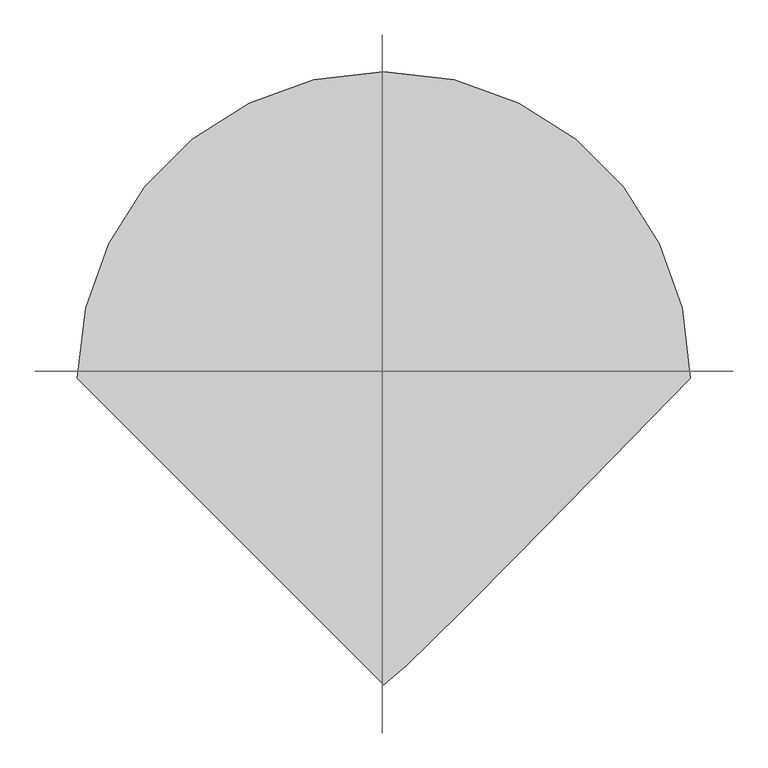
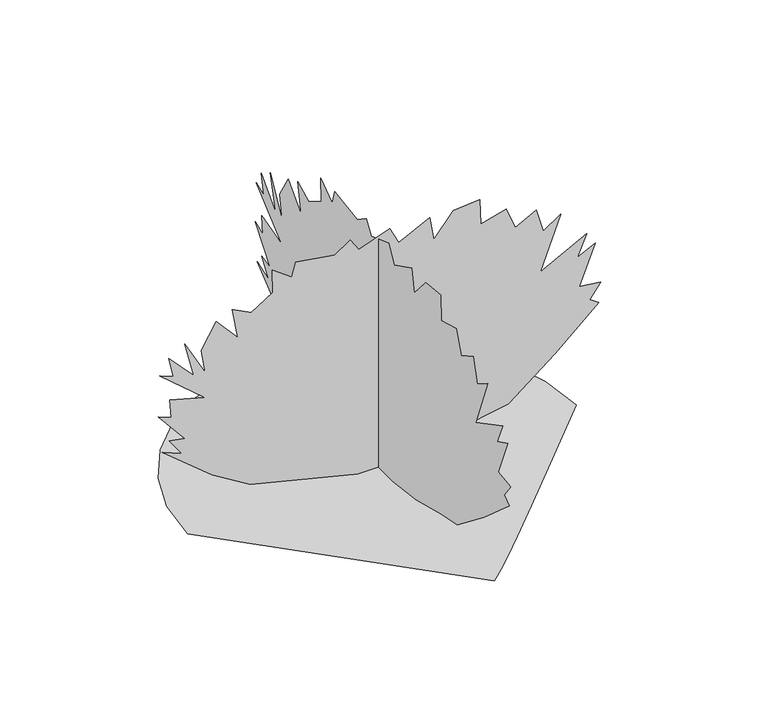
"""IFC4 building model written with IfcOpenShell, lengths in millimetres: proxy geometry, yew 26768 : yew 26768."""

from ifc_helpers import new_model, si_unit, origin, place, context, project, spatial, triangles, source, transform, mapped, element, save


def entourage_737b9002(model_context):
    return source(origin(), model_context, "Body", "Tessellation", [
        triangles([(-552.1733454, 0.0, 5.4e-06), (-537.5734008, 126.5215106, 5.4e-06), (-496.001229, 242.7110573, 5.4e-06), (-430.7790836, 345.2394648, 5.4e-06), (-345.2394648, 430.7790836, 5.4e-06), (-242.7110573, 496.001229, 5.4e-06), (-126.5212562, 537.5734008, 5.4e-06), (2.41e-05, 552.1733454, 5.4e-06), (126.5215106, 537.5734008, 5.4e-06), (242.7110573, 496.001229, 5.4e-06), (345.2394648, 430.7790836, 5.4e-06), (430.7790836, 345.2394648, 5.4e-06), (496.001229, 242.7110573, 5.4e-06), (537.5734008, 126.5212562, 5.4e-06), (552.1733454, -4.83e-05, 5.4e-06), (372.7273582, -184.0654909, 5.4e-06), (239.6978509, -319.5854711, 5.4e-06), (145.3449528, -414.6475465, 5.4e-06), (81.9343338, -477.3474621, 5.4e-06), (41.7301836, -515.775131, 5.4e-06), (16.9973058, -538.0179231, 5.4e-06), (-7.24e-05, -552.1733454, 5.4e-06), (-57.9623142, 12.396627, 5.21e-05), (-367.0047423, 12.396652, 75.5734076), (-474.5509031, 12.396652, 142.0056127), (-616.6665018, 12.396652, 259.1080397), (-561.3351408, 12.396652, 237.5164979), (-596.4227157, 12.396652, 287.4493694), (-553.2375973, 12.396652, 279.351844), (-628.8127808, 12.396652, 371.1195348), (-591.025189, 12.396652, 356.2757824), (-595.0739608, 12.396652, 410.2558814), (-496.5574814, 12.396652, 383.2658137), (-623.412747, 12.3966781, 491.2285552), (-585.6276987, 12.3966781, 476.3822594), (-597.7714342, 12.3966781, 535.7623921), (-527.5962845, 12.3966781, 460.1872087), (-553.2375973, 12.3966781, 564.1011784), (-495.2087265, 12.3966781, 457.4897352), (-506.0037435, 12.3966781, 527.6648849), (-464.1699234, 12.3966781, 599.1887532), (-402.0923172, 12.3966781, 530.3649018), (-418.2848245, 12.3966781, 619.4325394), (-364.3047255, 12.3966781, 591.091246), (-303.5758378, 12.3966781, 630.2275927), (-304.9245564, 12.3966781, 699.0539875), (-248.2454578, 12.3966781, 657.2201311), (-237.4491873, 12.3966781, 699.0539875), (-126.787955, 12.3966781, 681.5102182), (-82.2536094, 12.3966781, 711.2002665), (-57.9623142, 12.3966781, 673.4126747), (29.7568728, 12.3966781, 705.8027761), (55.3245209, 12.3966781, 655.0738958), (143.2032231, 12.3966781, 700.044552), (153.8874819, 12.3966781, 630.387612), (210.5935046, 12.3966781, 696.3564777), (284.8179166, 12.3966781, 704.4514778), (287.5154082, 12.3966781, 628.8788378), (360.3905748, 12.3966781, 649.1226603), (386.0318876, 12.3966781, 584.3450008), (445.4120204, 12.3966781, 616.7325588), (465.6532994, 12.3966781, 546.5574091), (515.5871701, 12.3966781, 578.9474742), (457.5557559, 12.396652, 426.4509321), (589.8110916, 12.3966781, 495.2747835), (562.8184805, 12.396652, 433.197141), (614.1011061, 12.3966781, 457.4897352), (568.2185143, 12.396652, 344.1295034), (628.9474382, 12.396652, 336.0319599), (597.9085988, 12.396652, 294.1956146), (623.5474045, 12.396652, 275.3030723), (498.0433645, 12.396652, 164.6420943), (365.7880651, 12.396652, 62.0781285), (289.9233281, 12.396652, 47.6486405), (164.5613216, 12.396652, 15.2766327), (36.5046395, 12.396627, 1.4e-05), (-3.3569921, 47.7068037, 4.09e-05), (-3.3569921, 356.74821, 75.5734076), (-3.3569921, 464.2969142, 142.0056127), (-3.3569921, 606.4099694, 259.1080397), (-3.3569921, 551.0786084, 237.5164979), (-3.3569921, 586.1687267, 287.4493694), (-3.3569921, 542.9836083, 279.351844), (-3.3569921, 618.5562847, 371.1195348), (-3.3569921, 580.7686566, 356.2757824), (-3.3569921, 584.8174284, 410.2558814), (-3.3569921, 486.3034925, 383.2658137), (-3.3569921, 613.1587944, 491.2285552), (-3.3569921, 575.3711663, 476.3822594), (-3.3569669, 587.5174453, 535.7623921), (-3.3569921, 517.3422956, 460.1872087), (-3.3569669, 542.9836083, 564.1011784), (-3.3569921, 484.9522305, 457.4897352), (-3.3569921, 495.7497545, 527.6648849), (-3.3569669, 453.913391, 599.1887532), (-3.3569921, 391.8357848, 530.3649018), (-3.3569669, 408.0308355, 619.4325394), (-3.3569921, 354.0481931, 591.091246), (-3.3569921, 293.3193054, 630.2275927), (-3.3569669, 294.6705856, 699.0539875), (-3.3569921, 237.9897067, 657.2201311), (-3.3569669, 227.1936905, 699.0539875), (-3.3569921, 116.5324491, 681.5102182), (-3.3569921, 71.9981035, 711.2002665), (-3.3569921, 47.7068037, 673.4126747), (-3.3569921, -40.0126331, 705.8027761), (-3.3569921, -65.5800314, 655.0738958), (-3.3569921, -153.458729, 700.044552), (-3.3569921, -164.1429969, 630.387612), (-3.3569921, -220.8490196, 696.3564777), (-3.3569921, -295.0719056, 704.4514778), (-3.3569921, -297.7719224, 628.8788378), (-3.3569921, -370.6471072, 649.1226603), (-3.3569921, -396.28842, 584.3450008), (-3.3569921, -455.6660093, 616.7325588), (-3.3569921, -475.9098318, 546.5574091), (-3.3569921, -525.8411591, 578.9474742), (-3.3569921, -467.8122883, 426.4509321), (-3.3569921, -600.0650442, 495.2747835), (-3.3569921, -573.0750129, 433.197141), (-3.3569921, -624.3576021, 457.4897352), (-3.3569921, -578.4725032, 344.1295034), (-3.3569921, -639.2013908, 336.0319599), (-3.3569921, -608.1625877, 294.1956146), (-3.3569921, -633.8039005, 275.3030723), (-3.3570177, -508.2973535, 164.6420943), (-3.3570177, -376.0445975, 62.0781285), (-3.3570177, -300.1798423, 47.6486405), (-3.3569921, -174.8168366, 15.2766327), (-3.3569921, -46.7601454, 0.0)], [[22, 21, 1], [21, 20, 1], [20, 19, 1], [19, 18, 1], [18, 17, 1], [1, 17, 2], [2, 17, 3], [3, 17, 4], [17, 16, 4], [4, 16, 5], [5, 16, 6], [6, 16, 7], [7, 16, 8], [8, 16, 9], [9, 16, 10], [10, 16, 11], [11, 16, 12], [16, 15, 12], [15, 14, 12], [14, 13, 12], [38, 37, 39], [26, 25, 27], [34, 33, 35], [30, 29, 31], [36, 35, 37], [35, 33, 37], [63, 62, 64], [65, 64, 66], [67, 66, 68], [28, 27, 29], [43, 42, 44], [46, 45, 47], [69, 68, 70], [37, 33, 39], [32, 31, 33], [54, 53, 55], [41, 40, 42], [61, 60, 62], [71, 70, 72], [31, 29, 33], [40, 39, 42], [57, 56, 58], [50, 49, 51], [56, 55, 58], [66, 64, 68], [48, 47, 49], [59, 58, 60], [52, 51, 53], [62, 60, 64], [70, 68, 72], [68, 64, 72], [72, 64, 73], [73, 64, 74], [27, 25, 29], [29, 25, 33], [25, 24, 33], [24, 23, 33], [74, 64, 75], [64, 60, 75], [60, 58, 75], [58, 55, 75], [75, 55, 76], [55, 53, 76], [76, 53, 23], [23, 53, 33], [53, 51, 33], [51, 49, 33], [49, 47, 33], [47, 45, 33], [39, 33, 42], [33, 45, 42], [45, 44, 42], [92, 91, 93], [80, 79, 81], [88, 87, 89], [84, 83, 85], [90, 89, 91], [89, 87, 91], [117, 116, 118], [119, 118, 120], [121, 120, 122], [82, 81, 83], [97, 96, 98], [100, 99, 101], [123, 122, 124], [91, 87, 93], [86, 85, 87], [108, 107, 109], [95, 94, 96], [115, 114, 116], [125, 124, 126], [85, 83, 87], [94, 93, 96], [111, 110, 112], [104, 103, 105], [110, 109, 112], [120, 118, 122], [102, 101, 103], [113, 112, 114], [106, 105, 107], [116, 114, 118], [124, 122, 126], [122, 118, 126], [126, 118, 127], [127, 118, 128], [81, 79, 83], [83, 79, 87], [79, 78, 87], [78, 77, 87], [128, 118, 129], [118, 114, 129], [114, 112, 129], [112, 109, 129], [129, 109, 130], [109, 107, 130], [130, 107, 77], [77, 107, 87], [107, 105, 87], [105, 103, 87], [103, 101, 87], [101, 99, 87], [93, 87, 96], [87, 99, 96], [99, 98, 96]], closed=False),
    ])


if __name__ == "__main__":
    model = new_model("IFC4")
    model_context = context("Model", 3, world=origin())
    ifc_project = project(units=[si_unit("LENGTHUNIT", "METRE", prefix="MILLI")], contexts=[model_context])
    site = spatial("IfcSite", under=ifc_project)
    building = spatial("IfcBuilding", under=site)
    placement = place(None, origin())
    entourage_shape = entourage_737b9002(model_context)
    element("IfcBuildingElementProxy", 1, Name="yew 26768 : yew 26768", ObjectType="yew 26768 : yew 26768", at=placement, inside=building, context=model_context, shape_type="MappedRepresentation", body=[
        mapped(entourage_shape, transform((0.0, 0.0, 0.0), x_axis=(1.0, 0.0, 0.0), y_axis=(0.0, 1.0, 0.0), z_axis=(0.0, 0.0, 1.0))),
    ])
    save(model, "model.ifc")

# Revit data of these elements
# Type "yew 26768 : yew 26768"
#   built-in parameter 1005195 = "RPC-16-FWJ8-ELQ0-EHM0-2000-ST1L-LVER-AU"
#   Height = 0
